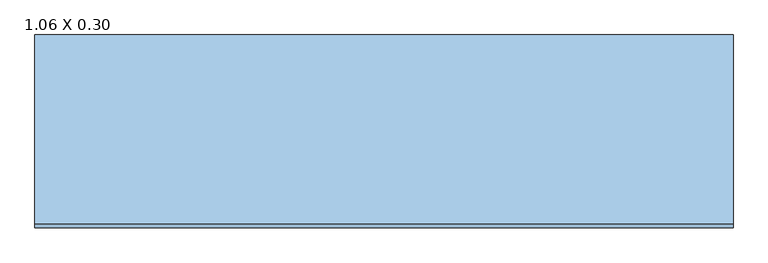
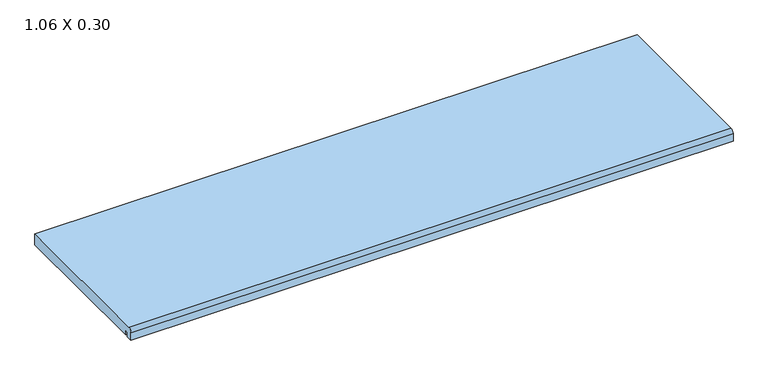
"""IFC4 building model written with IfcOpenShell, lengths in millimetres: window geometry, .CC_ND 300_PEDRA_PEITORIL RETO : 1.06 X 0.30."""

import ifcopenshell
import ifcopenshell.guid

model = None  # the IFC model being written
_history = None  # IfcOwnerHistory: only IFC2X3 demands one
_inside = {}  # id of a spatial element -> (the spatial element, [elements in it])
_under = {}  # id of a project, library or spatial element -> (it, [spatial elements below it])
_declared = {}  # id of a project -> (the project, [libraries it declares])
_typed = {}  # id of a type object -> (the type object, [elements of that type])
_made_of = {}  # id of a material, layer set ... -> (it, [elements and type objects made of it])


def new_model(schema):
    """Start an empty IFC model of exactly this schema.

    Asked for "IFC4X3", IfcOpenShell would pick the latest addendum, in which some entities
    have other attributes; the version numbers below select the first issue.
    IFC2X3 requires an IfcOwnerHistory on every rooted entity: one is made here for all.
    """
    global model, _history
    if schema == "IFC4X3":
        model = ifcopenshell.file(schema_version=(4, 3, 0, 0))
    else:
        model = ifcopenshell.file(schema=schema)
    _inside.clear()
    _under.clear()
    _declared.clear()
    _typed.clear()
    _made_of.clear()
    _history = None
    if model.schema == "IFC2X3":
        org = make("IfcOrganization", Name="unknown")
        user = make(
            "IfcPersonAndOrganization",
            ThePerson=make("IfcPerson", FamilyName="unknown"),
            TheOrganization=org,
        )
        app = make(
            "IfcApplication",
            ApplicationDeveloper=org,
            Version="unknown",
            ApplicationFullName="unknown",
            ApplicationIdentifier="unknown",
        )
        _history = make(
            "IfcOwnerHistory",
            OwningUser=user,
            OwningApplication=app,
            ChangeAction="ADDED",
            CreationDate=0,
        )
    return model


def make(cls, **values):
    """One entity of the class cls with the attributes given. An attribute that is None is left unset."""
    return model.create_entity(
        cls, **{name: value for name, value in values.items() if value is not None}
    )


def rooted(cls, **values):
    """An entity with a GlobalId (a new one), such as an element, a storey or a relation."""
    return make(cls, GlobalId=ifcopenshell.guid.new(), OwnerHistory=_history, **values)


def si_unit(unit_type, name, prefix=None):
    """IfcSIUnit, for example si_unit("LENGTHUNIT", "METRE", prefix="MILLI")."""
    return make("IfcSIUnit", UnitType=unit_type, Prefix=prefix, Name=name)


def assignment(units):
    """IfcUnitAssignment: the units of a project."""
    return None if units is None else make("IfcUnitAssignment", Units=units)


def point(xyz):
    """IfcCartesianPoint."""
    return None if xyz is None else make("IfcCartesianPoint", Coordinates=xyz)


def direction(xyz):
    """IfcDirection."""
    return None if xyz is None else make("IfcDirection", DirectionRatios=xyz)


def frame(location, z_axis=None, x_axis=None):
    """IfcAxis2Placement3D, a coordinate frame: its origin and axes. An axis left out is left unset."""
    return make(
        "IfcAxis2Placement3D",
        Location=point(location),
        Axis=direction(z_axis),
        RefDirection=direction(x_axis),
    )


def frame_2d(location, x_axis=None):
    """IfcAxis2Placement2D, a coordinate frame in the plane: its origin and x axis."""
    return make(
        "IfcAxis2Placement2D", Location=point(location), RefDirection=direction(x_axis)
    )


def origin():
    """The frame at (0, 0, 0) with its axes left unset."""
    return frame((0.0, 0.0, 0.0))


def place(relative_to, where):
    """IfcLocalPlacement: puts the frame where relative to a parent placement (None: the world)."""
    return make(
        "IfcLocalPlacement", PlacementRelTo=relative_to, RelativePlacement=where
    )


def context(
    kind, dimensions, precision=None, world=None, true_north=None, identifier=None
):
    """IfcGeometricRepresentationContext, for example the 3D "Model" context."""
    return make(
        "IfcGeometricRepresentationContext",
        ContextIdentifier=identifier,
        ContextType=kind,
        CoordinateSpaceDimension=dimensions,
        Precision=precision,
        WorldCoordinateSystem=world,
        TrueNorth=true_north,
    )


def project(units=None, contexts=None):
    """IfcProject with its units and contexts."""
    return rooted(
        "IfcProject",
        Name="project",
        RepresentationContexts=contexts,
        UnitsInContext=assignment(units),
    )


def spatial(cls, under=None, at=None, **own):
    """A site, building, storey or space (cls), placed at a placement, below another one or the project."""
    s = rooted(cls, ObjectPlacement=at, **own)
    if under is not None:
        _under.setdefault(under.id(), (under, []))[1].append(s)
    return s


def polyline(points):
    """IfcPolyline through the points."""
    return make("IfcPolyline", Points=[point(p) for p in points])


def circle_curve(where, radius):
    """IfcCircle in the frame where."""
    return make("IfcCircle", Position=where, Radius=radius)


def trimmed(basis, trim1, trim2, sense, master):
    """IfcTrimmedCurve: the piece of a basis curve between two trims."""
    return make(
        "IfcTrimmedCurve",
        BasisCurve=basis,
        Trim1=trim1,
        Trim2=trim2,
        SenseAgreement=sense,
        MasterRepresentation=master,
    )


def segment(curve, same_sense, transition):
    """IfcCompositeCurveSegment."""
    return make(
        "IfcCompositeCurveSegment",
        Transition=transition,
        SameSense=same_sense,
        ParentCurve=curve,
    )


def composite_curve(segments, self_intersect=None):
    """IfcCompositeCurve: segments joined end to end."""
    return make("IfcCompositeCurve", Segments=segments, SelfIntersect=self_intersect)


def outline(outer, holes=None, kind="AREA"):
    """IfcArbitraryClosedProfileDef: a profile drawn as a closed curve; with holes, ...WithVoids."""
    if holes is None:
        return make("IfcArbitraryClosedProfileDef", ProfileType=kind, OuterCurve=outer)
    return make(
        "IfcArbitraryProfileDefWithVoids",
        ProfileType=kind,
        OuterCurve=outer,
        InnerCurves=holes,
    )


def extrude(swept, where, along, depth):
    """IfcExtrudedAreaSolid: the profile swept, set in the frame where, extruded along a direction by depth."""
    return make(
        "IfcExtrudedAreaSolid",
        SweptArea=swept,
        Position=where,
        ExtrudedDirection=direction(along),
        Depth=depth,
    )


def shape(context_of_items, identifier, shape_type, items):
    """IfcShapeRepresentation: the items that make up one representation, for example the "Body"."""
    return make(
        "IfcShapeRepresentation",
        ContextOfItems=context_of_items,
        RepresentationIdentifier=identifier,
        RepresentationType=shape_type,
        Items=items,
    )


def source(mapping_origin, context_of_items, identifier, shape_type, items):
    """IfcRepresentationMap: a shape defined once, which mapped items show again and again."""
    return make(
        "IfcRepresentationMap",
        MappingOrigin=mapping_origin,
        MappedRepresentation=shape(context_of_items, identifier, shape_type, items),
    )


def transform(
    local_origin,
    x_axis=None,
    y_axis=None,
    z_axis=None,
    scale=None,
    scale2=None,
    scale3=None,
    uniform=True,
):
    """IfcCartesianTransformationOperator3D, or its non-uniform kind. x_axis, y_axis, z_axis: its Axis1, 2, 3."""
    if uniform:
        return make(
            "IfcCartesianTransformationOperator3D",
            Axis1=direction(x_axis),
            Axis2=direction(y_axis),
            LocalOrigin=point(local_origin),
            Scale=scale,
            Axis3=direction(z_axis),
        )
    return make(
        "IfcCartesianTransformationOperator3DnonUniform",
        Axis1=direction(x_axis),
        Axis2=direction(y_axis),
        LocalOrigin=point(local_origin),
        Scale=scale,
        Axis3=direction(z_axis),
        Scale2=scale2,
        Scale3=scale3,
    )


def mapped(mapping_source, mapping_target):
    """IfcMappedItem: shows the shape of a source again, moved by a transform."""
    return make(
        "IfcMappedItem", MappingSource=mapping_source, MappingTarget=mapping_target
    )


def made_of(thing, what):
    """Note that an element or type object is made of a material, layer set ...; save() writes the relation."""
    if what is not None:
        _made_of.setdefault(what.id(), (what, []))[1].append(thing)
    return thing


def element(
    cls,
    number,
    at=None,
    inside=None,
    cuts=None,
    type_object=None,
    material=None,
    context=None,
    identifier="Body",
    shape_type=None,
    held_by="IfcProductDefinitionShape",
    body=None,
    shapes=None,
    **own,
):
    """One element of the class cls, such as IfcWall. Its Tag is "e" and its number.

    at: its placement. inside: the storey or other place that contains it. cuts: it is an
    opening in that element (IfcRelVoidsElement). A single representation is given by context,
    identifier, shape_type and body (its items); several are given by shapes. held_by: the class
    of the entity that holds the representations. save() writes the other relations.
    """
    e = rooted(cls, Tag="e%d" % number, ObjectPlacement=at, **own)
    if body is not None:
        shapes = [shape(context, identifier, shape_type, body)]
    if shapes is not None:
        e.Representation = make(held_by, Representations=shapes)
    if inside is not None:
        _inside.setdefault(inside.id(), (inside, []))[1].append(e)
    if cuts is not None:
        rooted(
            "IfcRelVoidsElement", RelatingBuildingElement=cuts, RelatedOpeningElement=e
        )
    if type_object is not None:
        _typed.setdefault(type_object.id(), (type_object, []))[1].append(e)
    return made_of(e, material)


def aggregate(whole, parts):
    """IfcRelAggregates: a whole, such as a stair, and the parts it consists of."""
    return rooted("IfcRelAggregates", RelatingObject=whole, RelatedObjects=parts)


def save(model, path):
    """Write the relations noted so far, then the file.

    IfcRelAggregates (storeys below a building ...), IfcRelContainedInSpatialStructure (elements
    in a storey), IfcRelDefinesByType, IfcRelAssociatesMaterial and IfcRelDeclares: one each for
    every whole, place, type object, material and project.
    """
    for whole, parts in _under.values():
        aggregate(whole, parts)
    for where, things in _inside.values():
        rooted(
            "IfcRelContainedInSpatialStructure",
            RelatedElements=things,
            RelatingStructure=where,
        )
    for kind, things in _typed.values():
        rooted("IfcRelDefinesByType", RelatedObjects=things, RelatingType=kind)
    for what, things in _made_of.values():
        rooted("IfcRelAssociatesMaterial", RelatedObjects=things, RelatingMaterial=what)
    for by, libraries in _declared.values():
        rooted("IfcRelDeclares", RelatingContext=by, RelatedDefinitions=libraries)
    model.write(path)


def window_1_06_x_0_30_49639a84(model_context):
    return source(origin(), model_context, "Body", "SweptSolid", [
        extrude(outline(composite_curve([segment(polyline([(-132.5083081, 1480.0), (-132.5083081, 1488.1993124), (-137.2619526, 1488.1993124), (-137.2619526, 1480.0), (-148.0, 1480.0), (-148.0, 1493.3808343)]), True, "CONTINUOUS"), segment(trimmed(circle_curve(frame_2d((-141.3808343, 1493.3808343)), 6.6191657), [point((-148.0, 1493.3808343))], [point((-141.3808343, 1500.0))], False, "CARTESIAN"), True, "CONTINUOUS"), segment(polyline([(-141.3808343, 1500.0), (145.0, 1500.0), (145.0, 1480.0), (-132.5083081, 1480.0)]), True, "CONTINUOUS")], self_intersect=False)), frame((-530.0, 0.0, 0.0), z_axis=(1.0, 0.0, 0.0), x_axis=(0.0, 1.0, 0.0)), (0.0, 0.0, 1.0), 1060.0),
    ])


if __name__ == "__main__":
    model = new_model("IFC4")
    model_context = context("Model", 3, world=origin())
    ifc_project = project(units=[si_unit("LENGTHUNIT", "METRE", prefix="MILLI")], contexts=[model_context])
    site = spatial("IfcSite", under=ifc_project)
    building = spatial("IfcBuilding", under=site)
    placement = place(None, origin())
    window_1_06_x_0_30_shape = window_1_06_x_0_30_49639a84(model_context)
    element("IfcWindow", 1, ObjectType=".CC_ND 300_PEDRA_PEITORIL RETO : 1.06 X 0.30", at=placement, inside=building, context=model_context, shape_type="MappedRepresentation", body=[
        mapped(window_1_06_x_0_30_shape, transform((0.0, 0.0, 0.0), x_axis=(1.0, 0.0, 0.0), y_axis=(0.0, 1.0, 0.0), z_axis=(0.0, 0.0, 1.0))),
    ])
    save(model, "model.ifc")

# Revit data of these elements
# Type ".CC_ND 300_PEDRA_PEITORIL RETO : 1.06 X 0.30"
#   Type Mark = "68"
#   Largura da pedra [instance default] = 0.26 m
#   Extensão interior peitoril [instance default] = 0.03 m
#   Extensão exterior peitoril [instance default] = 0.03 m
#   Espessura = 0.02 m
#   Comprimento = 1.06 m
#   Altura-padrão do peitoril = 1.48 m
#   Peitoril = .GRANITO_BRANCO_ITAUNAS
#   Rough Width = 0
#   Rough Height = 0
#   Height = 0
#   Wall Closure = (empty or 0)
#   Width = 0
# Element 1 (IfcWindow, ".CC_ND 300_PEDRA_PEITORIL RETO : 1.06 X 0.30")
#   Largura da pedra = 0.293 m
#   Extensão interior peitoril = 0.027 m
#   Materials on its faces: ".GRANITO_BRANCO_ITAUNAS"
# Materials
#   ".GRANITO_BRANCO_ITAUNAS": class ".CC_PEDRA REVEST.", colour RGB 202 195 174, transparency 0, Description = "Revestimento em granito", Cost = 0
